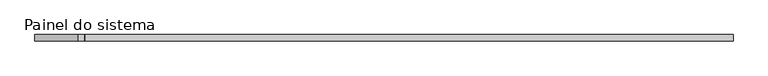
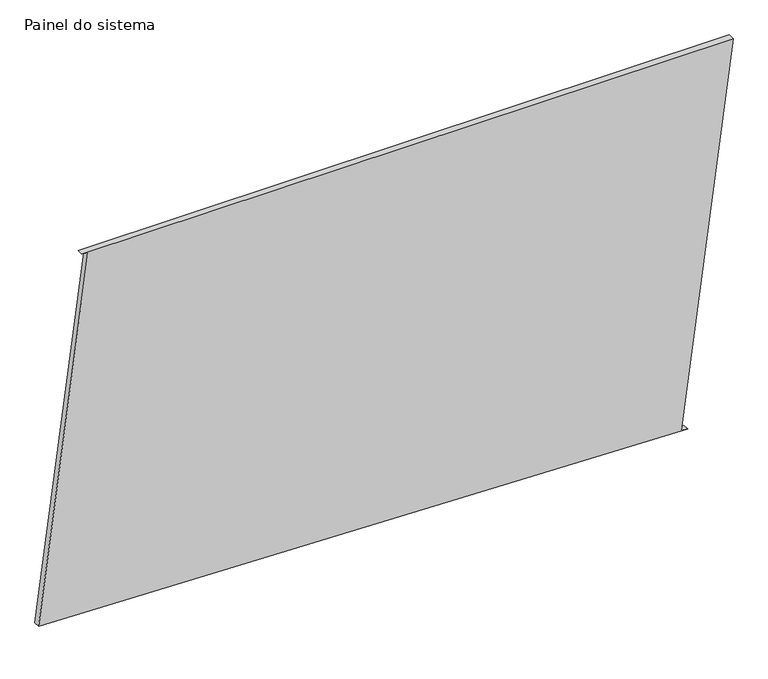
"""IFC4 building model written with IfcOpenShell, lengths in millimetres: plate geometry, Painel do sistema : Envidraçado."""

from ifc_helpers import new_model, si_unit, frame, origin, place, context, project, spatial, polyline, outline, extrude, source, transform, mapped, element, save


def painel_do_sistema_c9666536(model_context):
    return source(origin(), model_context, "Body", "SweptSolid", [
        extrude(outline(polyline([(0.0, 1190.1123692), (3.2380023, 1165.3229493), (1567.3179738, 1369.6235945), (1567.3179738, -1199.6468276), (1564.0799716, -1174.8574077), (72.9936776, -1369.6235945), (0.0, 1190.1123692)])), frame((0.0, 24.5, 0.0), z_axis=(0.0, 1.0, 0.0), x_axis=(0.0, 0.0, 1.0)), (0.0, 0.0, 1.0), 25.0),
    ])


if __name__ == "__main__":
    model = new_model("IFC4")
    model_context = context("Model", 3, world=origin())
    ifc_project = project(units=[si_unit("LENGTHUNIT", "METRE", prefix="MILLI")], contexts=[model_context])
    site = spatial("IfcSite", under=ifc_project)
    building = spatial("IfcBuilding", under=site)
    placement = place(None, origin())
    painel_do_sistema_shape = painel_do_sistema_c9666536(model_context)
    element("IfcPlate", 1, ObjectType="Painel do sistema : Envidraçado", at=placement, inside=building, context=model_context, shape_type="MappedRepresentation", body=[
        mapped(painel_do_sistema_shape, transform((0.0, 0.0, 0.0), x_axis=(1.0, 0.0, 0.0), y_axis=(0.0, 1.0, 0.0), z_axis=(0.0, 0.0, 1.0))),
    ])
    save(model, "model.ifc")

# Revit data of these elements
# Type "Painel do sistema : Envidraçado"
#   Construction Type Id = "GSP4R"
#   Analytic Construction = "Vidraça única Pilkington 1/8 pol"
#   Visual Light Transmittance = 0.9
#   Solar Heat Gain Coefficient = 0.86
#   Heat Transfer Coefficient (U) = 6.7069 W/(m²·K)
# Element 1 (IfcPlate, "Painel do sistema : Envidraçado")
#   Materials on its faces: "Vidro"
# Materials
#   "Vidro": class "Vidro", colour RGB 0 128 192, transparency 0.9, Description = "Vidro de sílica", Cost = 0
